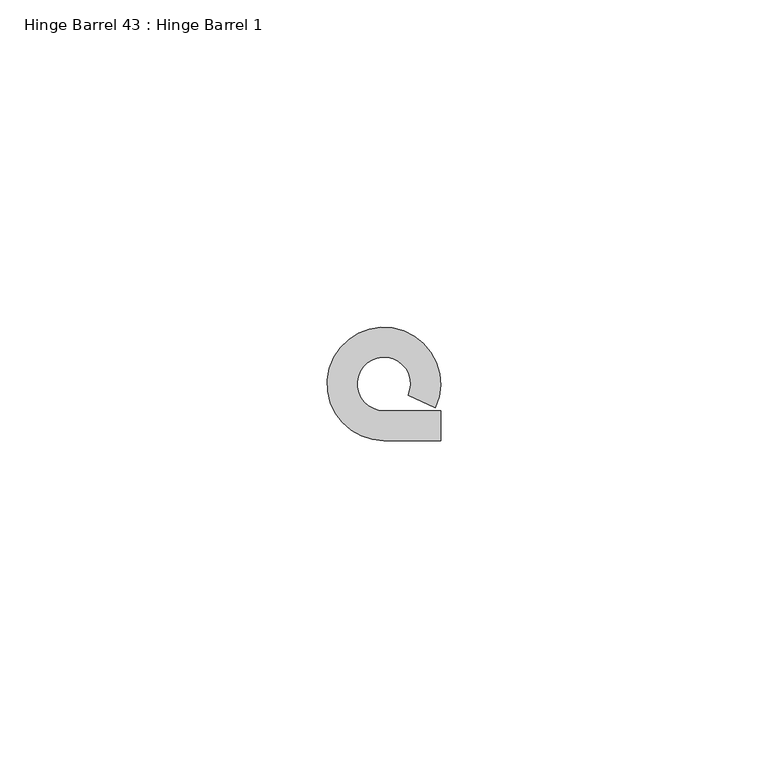
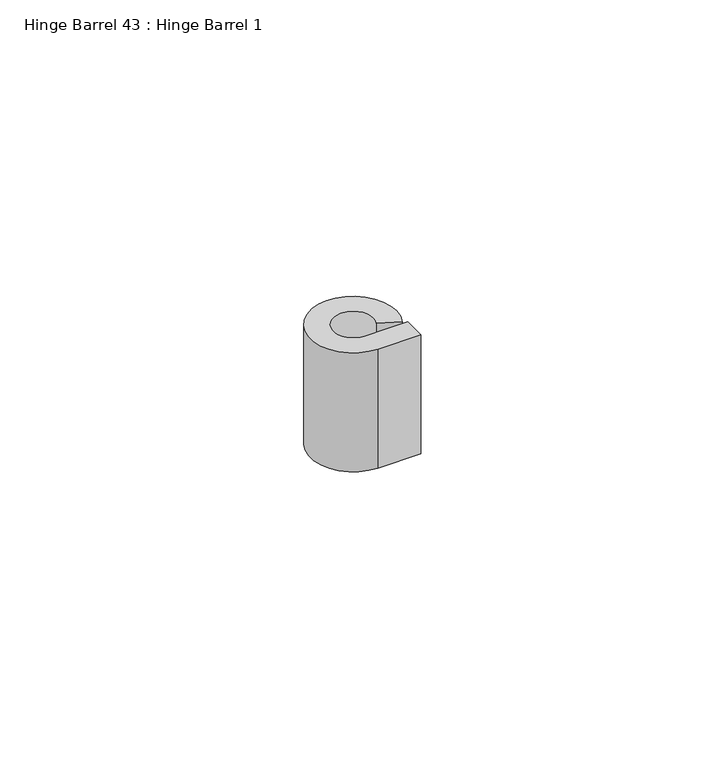
"""IFC4 building model written with IfcOpenShell, lengths in millimetres: proxy geometry, Hinge Barrel 43 : Hinge Barrel 1."""

import ifcopenshell
import ifcopenshell.guid

model = None  # the IFC model being written
_history = None  # IfcOwnerHistory: only IFC2X3 demands one
_inside = {}  # id of a spatial element -> (the spatial element, [elements in it])
_under = {}  # id of a project, library or spatial element -> (it, [spatial elements below it])
_declared = {}  # id of a project -> (the project, [libraries it declares])
_typed = {}  # id of a type object -> (the type object, [elements of that type])
_made_of = {}  # id of a material, layer set ... -> (it, [elements and type objects made of it])


def new_model(schema):
    """Start an empty IFC model of exactly this schema.

    Asked for "IFC4X3", IfcOpenShell would pick the latest addendum, in which some entities
    have other attributes; the version numbers below select the first issue.
    IFC2X3 requires an IfcOwnerHistory on every rooted entity: one is made here for all.
    """
    global model, _history
    if schema == "IFC4X3":
        model = ifcopenshell.file(schema_version=(4, 3, 0, 0))
    else:
        model = ifcopenshell.file(schema=schema)
    _inside.clear()
    _under.clear()
    _declared.clear()
    _typed.clear()
    _made_of.clear()
    _history = None
    if model.schema == "IFC2X3":
        org = make("IfcOrganization", Name="unknown")
        user = make(
            "IfcPersonAndOrganization",
            ThePerson=make("IfcPerson", FamilyName="unknown"),
            TheOrganization=org,
        )
        app = make(
            "IfcApplication",
            ApplicationDeveloper=org,
            Version="unknown",
            ApplicationFullName="unknown",
            ApplicationIdentifier="unknown",
        )
        _history = make(
            "IfcOwnerHistory",
            OwningUser=user,
            OwningApplication=app,
            ChangeAction="ADDED",
            CreationDate=0,
        )
    return model


def make(cls, **values):
    """One entity of the class cls with the attributes given. An attribute that is None is left unset."""
    return model.create_entity(
        cls, **{name: value for name, value in values.items() if value is not None}
    )


def rooted(cls, **values):
    """An entity with a GlobalId (a new one), such as an element, a storey or a relation."""
    return make(cls, GlobalId=ifcopenshell.guid.new(), OwnerHistory=_history, **values)


def si_unit(unit_type, name, prefix=None):
    """IfcSIUnit, for example si_unit("LENGTHUNIT", "METRE", prefix="MILLI")."""
    return make("IfcSIUnit", UnitType=unit_type, Prefix=prefix, Name=name)


def assignment(units):
    """IfcUnitAssignment: the units of a project."""
    return None if units is None else make("IfcUnitAssignment", Units=units)


def point(xyz):
    """IfcCartesianPoint."""
    return None if xyz is None else make("IfcCartesianPoint", Coordinates=xyz)


def direction(xyz):
    """IfcDirection."""
    return None if xyz is None else make("IfcDirection", DirectionRatios=xyz)


def frame(location, z_axis=None, x_axis=None):
    """IfcAxis2Placement3D, a coordinate frame: its origin and axes. An axis left out is left unset."""
    return make(
        "IfcAxis2Placement3D",
        Location=point(location),
        Axis=direction(z_axis),
        RefDirection=direction(x_axis),
    )


def frame_2d(location, x_axis=None):
    """IfcAxis2Placement2D, a coordinate frame in the plane: its origin and x axis."""
    return make(
        "IfcAxis2Placement2D", Location=point(location), RefDirection=direction(x_axis)
    )


def origin():
    """The frame at (0, 0, 0) with its axes left unset."""
    return frame((0.0, 0.0, 0.0))


def place(relative_to, where):
    """IfcLocalPlacement: puts the frame where relative to a parent placement (None: the world)."""
    return make(
        "IfcLocalPlacement", PlacementRelTo=relative_to, RelativePlacement=where
    )


def context(
    kind, dimensions, precision=None, world=None, true_north=None, identifier=None
):
    """IfcGeometricRepresentationContext, for example the 3D "Model" context."""
    return make(
        "IfcGeometricRepresentationContext",
        ContextIdentifier=identifier,
        ContextType=kind,
        CoordinateSpaceDimension=dimensions,
        Precision=precision,
        WorldCoordinateSystem=world,
        TrueNorth=true_north,
    )


def project(units=None, contexts=None):
    """IfcProject with its units and contexts."""
    return rooted(
        "IfcProject",
        Name="project",
        RepresentationContexts=contexts,
        UnitsInContext=assignment(units),
    )


def spatial(cls, under=None, at=None, **own):
    """A site, building, storey or space (cls), placed at a placement, below another one or the project."""
    s = rooted(cls, ObjectPlacement=at, **own)
    if under is not None:
        _under.setdefault(under.id(), (under, []))[1].append(s)
    return s


def polyline(points):
    """IfcPolyline through the points."""
    return make("IfcPolyline", Points=[point(p) for p in points])


def circle_curve(where, radius):
    """IfcCircle in the frame where."""
    return make("IfcCircle", Position=where, Radius=radius)


def trimmed(basis, trim1, trim2, sense, master):
    """IfcTrimmedCurve: the piece of a basis curve between two trims."""
    return make(
        "IfcTrimmedCurve",
        BasisCurve=basis,
        Trim1=trim1,
        Trim2=trim2,
        SenseAgreement=sense,
        MasterRepresentation=master,
    )


def segment(curve, same_sense, transition):
    """IfcCompositeCurveSegment."""
    return make(
        "IfcCompositeCurveSegment",
        Transition=transition,
        SameSense=same_sense,
        ParentCurve=curve,
    )


def composite_curve(segments, self_intersect=None):
    """IfcCompositeCurve: segments joined end to end."""
    return make("IfcCompositeCurve", Segments=segments, SelfIntersect=self_intersect)


def outline(outer, holes=None, kind="AREA"):
    """IfcArbitraryClosedProfileDef: a profile drawn as a closed curve; with holes, ...WithVoids."""
    if holes is None:
        return make("IfcArbitraryClosedProfileDef", ProfileType=kind, OuterCurve=outer)
    return make(
        "IfcArbitraryProfileDefWithVoids",
        ProfileType=kind,
        OuterCurve=outer,
        InnerCurves=holes,
    )


def extrude(swept, where, along, depth):
    """IfcExtrudedAreaSolid: the profile swept, set in the frame where, extruded along a direction by depth."""
    return make(
        "IfcExtrudedAreaSolid",
        SweptArea=swept,
        Position=where,
        ExtrudedDirection=direction(along),
        Depth=depth,
    )


def shape(context_of_items, identifier, shape_type, items):
    """IfcShapeRepresentation: the items that make up one representation, for example the "Body"."""
    return make(
        "IfcShapeRepresentation",
        ContextOfItems=context_of_items,
        RepresentationIdentifier=identifier,
        RepresentationType=shape_type,
        Items=items,
    )


def source(mapping_origin, context_of_items, identifier, shape_type, items):
    """IfcRepresentationMap: a shape defined once, which mapped items show again and again."""
    return make(
        "IfcRepresentationMap",
        MappingOrigin=mapping_origin,
        MappedRepresentation=shape(context_of_items, identifier, shape_type, items),
    )


def transform(
    local_origin,
    x_axis=None,
    y_axis=None,
    z_axis=None,
    scale=None,
    scale2=None,
    scale3=None,
    uniform=True,
):
    """IfcCartesianTransformationOperator3D, or its non-uniform kind. x_axis, y_axis, z_axis: its Axis1, 2, 3."""
    if uniform:
        return make(
            "IfcCartesianTransformationOperator3D",
            Axis1=direction(x_axis),
            Axis2=direction(y_axis),
            LocalOrigin=point(local_origin),
            Scale=scale,
            Axis3=direction(z_axis),
        )
    return make(
        "IfcCartesianTransformationOperator3DnonUniform",
        Axis1=direction(x_axis),
        Axis2=direction(y_axis),
        LocalOrigin=point(local_origin),
        Scale=scale,
        Axis3=direction(z_axis),
        Scale2=scale2,
        Scale3=scale3,
    )


def mapped(mapping_source, mapping_target):
    """IfcMappedItem: shows the shape of a source again, moved by a transform."""
    return make(
        "IfcMappedItem", MappingSource=mapping_source, MappingTarget=mapping_target
    )


def made_of(thing, what):
    """Note that an element or type object is made of a material, layer set ...; save() writes the relation."""
    if what is not None:
        _made_of.setdefault(what.id(), (what, []))[1].append(thing)
    return thing


def element(
    cls,
    number,
    at=None,
    inside=None,
    cuts=None,
    type_object=None,
    material=None,
    context=None,
    identifier="Body",
    shape_type=None,
    held_by="IfcProductDefinitionShape",
    body=None,
    shapes=None,
    **own,
):
    """One element of the class cls, such as IfcWall. Its Tag is "e" and its number.

    at: its placement. inside: the storey or other place that contains it. cuts: it is an
    opening in that element (IfcRelVoidsElement). A single representation is given by context,
    identifier, shape_type and body (its items); several are given by shapes. held_by: the class
    of the entity that holds the representations. save() writes the other relations.
    """
    e = rooted(cls, Tag="e%d" % number, ObjectPlacement=at, **own)
    if body is not None:
        shapes = [shape(context, identifier, shape_type, body)]
    if shapes is not None:
        e.Representation = make(held_by, Representations=shapes)
    if inside is not None:
        _inside.setdefault(inside.id(), (inside, []))[1].append(e)
    if cuts is not None:
        rooted(
            "IfcRelVoidsElement", RelatingBuildingElement=cuts, RelatedOpeningElement=e
        )
    if type_object is not None:
        _typed.setdefault(type_object.id(), (type_object, []))[1].append(e)
    return made_of(e, material)


def aggregate(whole, parts):
    """IfcRelAggregates: a whole, such as a stair, and the parts it consists of."""
    return rooted("IfcRelAggregates", RelatingObject=whole, RelatedObjects=parts)


def save(model, path):
    """Write the relations noted so far, then the file.

    IfcRelAggregates (storeys below a building ...), IfcRelContainedInSpatialStructure (elements
    in a storey), IfcRelDefinesByType, IfcRelAssociatesMaterial and IfcRelDeclares: one each for
    every whole, place, type object, material and project.
    """
    for whole, parts in _under.values():
        aggregate(whole, parts)
    for where, things in _inside.values():
        rooted(
            "IfcRelContainedInSpatialStructure",
            RelatedElements=things,
            RelatingStructure=where,
        )
    for kind, things in _typed.values():
        rooted("IfcRelDefinesByType", RelatedObjects=things, RelatingType=kind)
    for what, things in _made_of.values():
        rooted("IfcRelAssociatesMaterial", RelatedObjects=things, RelatingMaterial=what)
    for by, libraries in _declared.values():
        rooted("IfcRelDeclares", RelatingContext=by, RelatedDefinitions=libraries)
    model.write(path)


def hinge_barrel_43_hinge_barrel_1_81794a76(model_context):
    return source(origin(), model_context, "Body", "SweptSolid", [
        extrude(outline(composite_curve([segment(polyline([(587323.2214739, -534104.7943841), (587327.7934739, -534104.7943841), (587327.7934739, -534109.3584466), (587319.1320739, -534109.3584466)]), True, "CONTINUOUS"), segment(trimmed(circle_curve(frame_2d((587319.1320739, -534100.7049841)), 8.6534625), [point((587319.1320739, -534109.3584466))], [point((587326.986084, -534104.3377433))], False, "CARTESIAN"), True, "CONTINUOUS"), segment(polyline([(587326.986084, -534104.3377433), (587322.8436736, -534102.421731)]), True, "CONTINUOUS"), segment(trimmed(circle_curve(frame_2d((587319.1320739, -534100.7049841)), 4.0894), [point((587322.8436736, -534102.421731))], [point((587319.1320739, -534104.7943841))], True, "CARTESIAN"), True, "CONTINUOUS"), segment(polyline([(587319.1320739, -534104.7943841), (587323.2214739, -534104.7943841)]), True, "CONTINUOUS")], self_intersect=False)), frame((0.0, 0.0, 1936.75), z_axis=(0.0, 0.0, 1.0), x_axis=(1.0, 0.0, 0.0)), (0.0, 0.0, 1.0), 25.4),
    ])


if __name__ == "__main__":
    model = new_model("IFC4")
    model_context = context("Model", 3, world=origin())
    ifc_project = project(units=[si_unit("LENGTHUNIT", "METRE", prefix="MILLI")], contexts=[model_context])
    site = spatial("IfcSite", under=ifc_project)
    building = spatial("IfcBuilding", under=site)
    placement = place(None, origin())
    hinge_barrel_43_hinge_barrel_1_shape = hinge_barrel_43_hinge_barrel_1_81794a76(model_context)
    element("IfcBuildingElementProxy", 1, Name="Hinge Barrel 43 : Hinge Barrel 1", ObjectType="Hinge Barrel 43 : Hinge Barrel 1", at=placement, inside=building, context=model_context, shape_type="MappedRepresentation", body=[
        mapped(hinge_barrel_43_hinge_barrel_1_shape, transform((0.0, 0.0, 0.0), x_axis=(1.0, 0.0, 0.0), y_axis=(0.0, 1.0, 0.0), z_axis=(0.0, 0.0, 1.0))),
    ])
    save(model, "model.ifc")

# Revit data of these elements
# Element 1 (IfcBuildingElementProxy, "Hinge Barrel 43 : Hinge Barrel 1")
#   Materials on its faces: "6\"X6\" WELD-ON STL BUTT HINGE"
# Materials
#   "6\"X6\" WELD-ON STL BUTT HINGE": class "Metal", colour RGB 189 187 185, transparency 0, Description = "Carbon steel", Cost = 0
